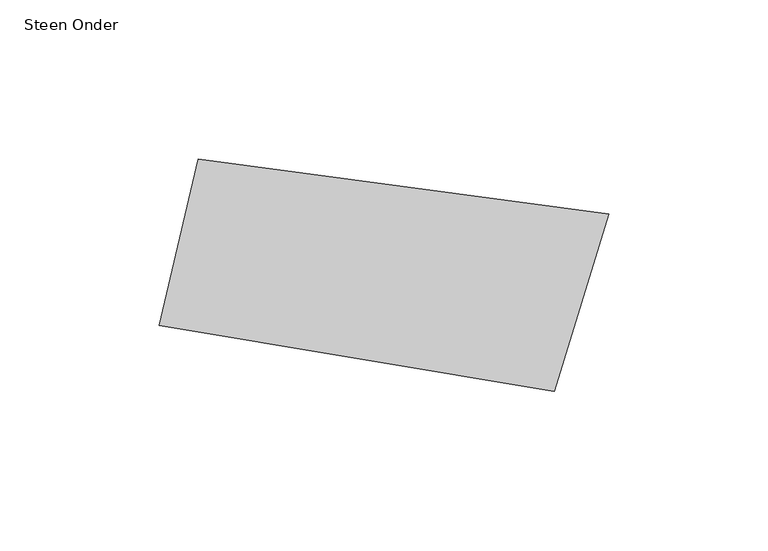
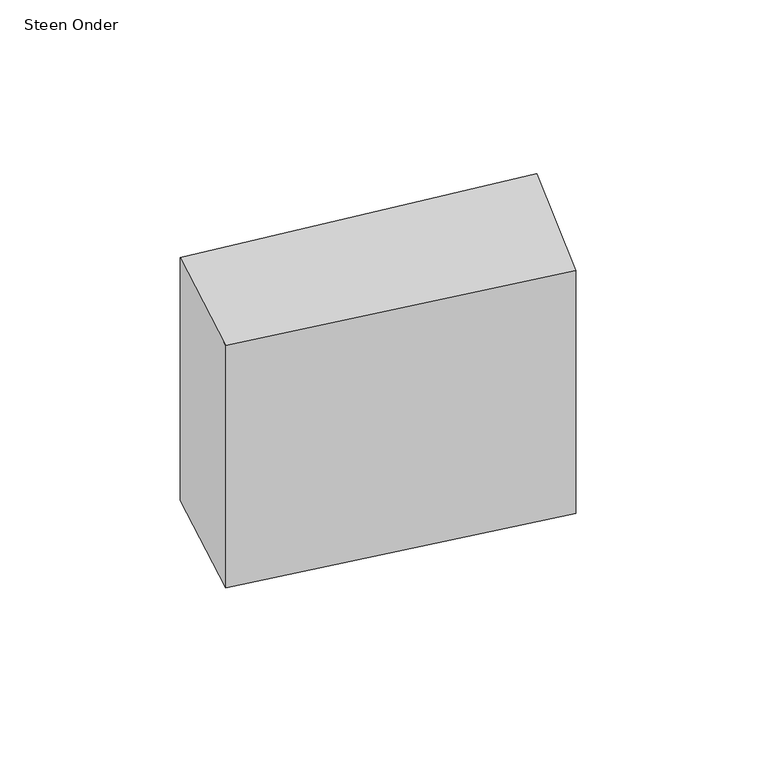
"""IFC4 building model written with IfcOpenShell, lengths in millimetres: proxy geometry, 00_GMA_steen_versie_4 : Steen Onder."""

from ifc_helpers import new_model, si_unit, frame, origin, place, context, project, spatial, polyline, outline, extrude, source, transform, mapped, element, save


def steen_onder_dc579bc1(model_context):
    return source(origin(), model_context, "Body", "SweptSolid", [
        extrude(outline(polyline([(166.4091508, 55.4140748), (149.2937686, -0.433256), (25.0980818, 20.428799), (37.4621162, 72.7223919), (166.4091508, 55.4140748)])), frame((0.0, 0.0, -100.0), z_axis=(0.0, 0.0, 1.0), x_axis=(1.0, 0.0, 0.0)), (0.0, 0.0, 1.0), 100.0),
    ])


if __name__ == "__main__":
    model = new_model("IFC4")
    model_context = context("Model", 3, world=origin())
    ifc_project = project(units=[si_unit("LENGTHUNIT", "METRE", prefix="MILLI")], contexts=[model_context])
    site = spatial("IfcSite", under=ifc_project)
    building = spatial("IfcBuilding", under=site)
    placement = place(None, origin())
    steen_onder_shape = steen_onder_dc579bc1(model_context)
    element("IfcBuildingElementProxy", 1, Name="00_GMA_steen_versie_4 : Steen Onder", ObjectType="00_GMA_steen_versie_4 : Steen Onder", at=placement, inside=building, context=model_context, shape_type="MappedRepresentation", body=[
        mapped(steen_onder_shape, transform((0.0, 0.0, 0.0), x_axis=(1.0, 0.0, 0.0), y_axis=(0.0, 1.0, 0.0), z_axis=(0.0, 0.0, 1.0))),
    ])
    save(model, "model.ifc")

# Revit data of these elements
# Type "00_GMA_steen_versie_4 : Steen Onder"
#   StootVoegHalfBoven [instance default] = 5 mm
#   StootVoegHalf [instance default] = 5 mm
#   StootVoegBreedteOnder = 10 mm
#   StootVoegBreedteBoven = 10 mm
#   Steendikte = 100 mm
#   LintVoegOnderHalf = 0 mm
#   LintVoegOnder = 0 mm
#   LintVoegBovenHalf = 5 mm
#   LintVoegBoven = 10 mm
#   materiaal = none
#   MateriaalVoeg = none
#   Default Elevation = 0
